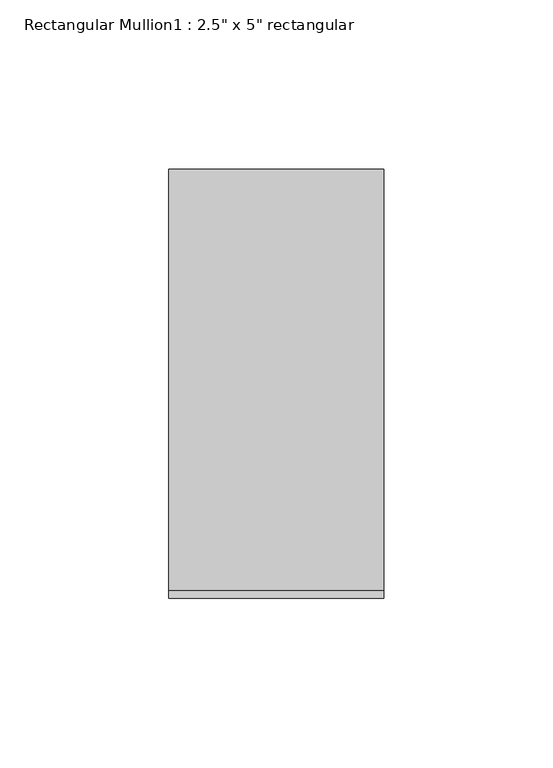
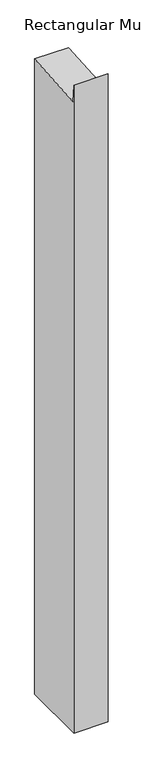
"""IFC4 building model written with IfcOpenShell, lengths in millimetres: member geometry."""

from ifc_helpers import new_model, si_unit, frame, origin, place, context, project, spatial, polyline, outline, extrude, source, transform, mapped, element, save


def member_fbb04c12(model_context):
    return source(origin(), model_context, "Body", "SweptSolid", [
        extrude(outline(polyline([(-63.5, 29.5516342), (-61.1522336, -4.315452), (63.5, 4.3258089), (63.5, -1249.2609667), (-63.5, -1249.2609667), (-63.5, 29.5516342)])), frame((-63.5, 0.0, 0.0), z_axis=(1.0, 0.0, 0.0), x_axis=(0.0, 1.0, 0.0)), (0.0, 0.0, 1.0), 63.5),
    ])


if __name__ == "__main__":
    model = new_model("IFC4")
    model_context = context("Model", 3, world=origin())
    ifc_project = project(units=[si_unit("LENGTHUNIT", "METRE", prefix="MILLI")], contexts=[model_context])
    site = spatial("IfcSite", under=ifc_project)
    building = spatial("IfcBuilding", under=site)
    placement = place(None, origin())
    member_shape = member_fbb04c12(model_context)
    element("IfcMember", 1, ObjectType="Rectangular Mullion1 : 2.5\" x 5\" rectangular", at=placement, inside=building, context=model_context, shape_type="MappedRepresentation", body=[
        mapped(member_shape, transform((0.0, 0.0, 0.0), x_axis=(1.0, 0.0, 0.0), y_axis=(0.0, 1.0, 0.0), z_axis=(0.0, 0.0, 1.0))),
    ])
    save(model, "model.ifc")

# Revit data of these elements
# Type "Rectangular Mullion1 : 2.5\" x 5\" rectangular"
#   built-in parameter 1007304 = 0.416667 (stored number, unit not read)
#   built-in parameter 1007301 = 0.104167 (stored number, unit not read)
#   built-in parameter 1007300 = 0.104167 (stored number, unit not read)
# Element 1 (IfcMember, "Rectangular Mullion1 : 2.5\" x 5\" rectangular")
#   Materials on its faces: "support-frame"
# Materials
#   "support-frame": class "Unassigned", colour RGB 233 233 233, transparency 0, Cost = 0
